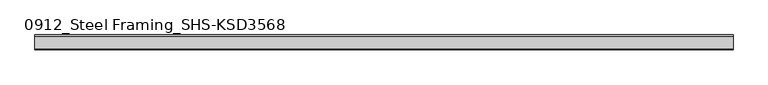
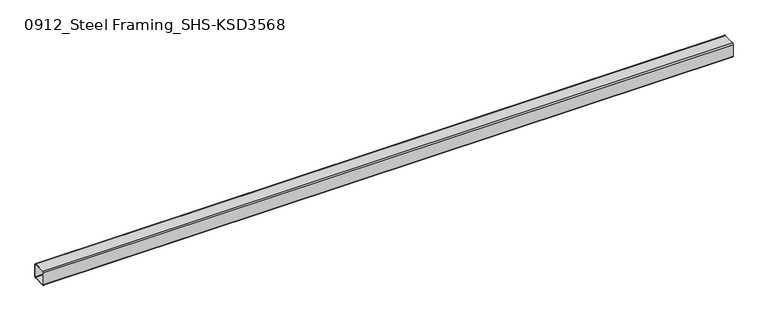
"""IFC4 building model written with IfcOpenShell, lengths in millimetres: beam geometry, 0912_Steel Framing_SHS-KSD3568 : H_SB_ASB_SHS-150x150x6."""

from ifc_helpers import new_model, si_unit, point, frame, frame_2d, origin, place, context, project, spatial, polyline, circle_curve, trimmed, segment, composite_curve, outline, extrude, source, transform, mapped, element, save


def beam_0912_steel_framing_shs_ksd3568_74c151f8(model_context):
    return source(origin(), model_context, "Body", "SweptSolid", [
        extrude(outline(composite_curve([segment(polyline([(75.0, 63.0), (75.0, -63.0)]), True, "CONTINUOUS"), segment(trimmed(circle_curve(frame_2d((63.0, -63.0)), 12.0), [point((75.0, -63.0))], [point((63.0, -75.0))], False, "CARTESIAN"), True, "CONTINUOUS"), segment(polyline([(63.0, -75.0), (-63.0, -75.0)]), True, "CONTINUOUS"), segment(trimmed(circle_curve(frame_2d((-63.0, -63.0)), 12.0), [point((-63.0, -75.0))], [point((-75.0, -63.0))], False, "CARTESIAN"), True, "CONTINUOUS"), segment(polyline([(-75.0, -63.0), (-75.0, 63.0)]), True, "CONTINUOUS"), segment(trimmed(circle_curve(frame_2d((-63.0, 63.0)), 12.0), [point((-75.0, 63.0))], [point((-63.0, 75.0))], False, "CARTESIAN"), True, "CONTINUOUS"), segment(polyline([(-63.0, 75.0), (63.0, 75.0)]), True, "CONTINUOUS"), segment(trimmed(circle_curve(frame_2d((63.0, 63.0)), 12.0), [point((63.0, 75.0))], [point((75.0, 63.0))], False, "CARTESIAN"), True, "CONTINUOUS")], self_intersect=False), holes=[composite_curve([segment(trimmed(circle_curve(frame_2d((-63.0, 63.0)), 6.0), [point((-63.0, 69.0))], [point((-69.0, 63.0))], True, "CARTESIAN"), True, "CONTINUOUS"), segment(polyline([(-69.0, 63.0), (-69.0, -63.0)]), True, "CONTINUOUS"), segment(trimmed(circle_curve(frame_2d((-63.0, -63.0)), 6.0), [point((-69.0, -63.0))], [point((-63.0, -69.0))], True, "CARTESIAN"), True, "CONTINUOUS"), segment(polyline([(-63.0, -69.0), (63.0, -69.0)]), True, "CONTINUOUS"), segment(trimmed(circle_curve(frame_2d((63.0, -63.0)), 6.0), [point((63.0, -69.0))], [point((69.0, -63.0))], True, "CARTESIAN"), True, "CONTINUOUS"), segment(polyline([(69.0, -63.0), (69.0, 63.0)]), True, "CONTINUOUS"), segment(trimmed(circle_curve(frame_2d((63.0, 63.0)), 6.0), [point((69.0, 63.0))], [point((63.0, 69.0))], True, "CARTESIAN"), True, "CONTINUOUS"), segment(polyline([(63.0, 69.0), (-63.0, 69.0)]), True, "CONTINUOUS")], self_intersect=False)]), frame((-3490.0, 0.0, 0.0), z_axis=(1.0, 0.0, 0.0), x_axis=(0.0, 1.0, 0.0)), (0.0, 0.0, 1.0), 6980.0),
    ])


if __name__ == "__main__":
    model = new_model("IFC4")
    model_context = context("Model", 3, world=origin())
    ifc_project = project(units=[si_unit("LENGTHUNIT", "METRE", prefix="MILLI")], contexts=[model_context])
    site = spatial("IfcSite", under=ifc_project)
    building = spatial("IfcBuilding", under=site)
    placement = place(None, origin())
    beam_0912_steel_framing_shs_ksd3568_shape = beam_0912_steel_framing_shs_ksd3568_74c151f8(model_context)
    element("IfcBeam", 1, ObjectType="0912_Steel Framing_SHS-KSD3568 : H_SB_ASB_SHS-150x150x6", at=placement, inside=building, context=model_context, shape_type="MappedRepresentation", body=[
        mapped(beam_0912_steel_framing_shs_ksd3568_shape, transform((0.0, 0.0, 0.0), x_axis=(1.0, 0.0, 0.0), y_axis=(0.0, 1.0, 0.0), z_axis=(0.0, 0.0, 1.0))),
    ])
    save(model, "model.ifc")

# Revit data of these elements
# Type "0912_Steel Framing_SHS-KSD3568 : H_SB_ASB_SHS-150x150x6"
#   H_WM Code_1 = "S01AA002-00001 | Main Steel Structure Fabrication Work | Shelter/Building | Medium Steel - Standard (90KG/M>Weight≥30KG/M) | Material: (   )"
#   H_WM Code_2 = "S03AA028-00001 | Main Steel Structure Erection Work | Shelter/Building | Medium Steel (90KG/M>Weight≥30KG/M) | Material: (   )"
#   H_WM Code_3 = "S01AA010-00001 | Main Steel Structure Fabrication Work | Shelter/Building | Steel Painting/Coating | for Non-Fireproofed Steel Surface, Surface Preparation, Primer, Second & Final Coat | Material: (   )"
#   H_Q'ty Cal Type Tag = "SB-Q2"
#   Perimeter = 0.60 m²/m
#   Nominal Weight = 26.40 kgf/m
#   Length [instance default] = 1.0000 m
#   b = 0.1500 m
#   h = 0.1500 m
#   tr = 0.0120 m
#   t = 0.0060 m
#   A = 28.36 m²
#   Structural Material [instance default] = Steel, 45-345
# Element 1 (IfcBeam, "0912_Steel Framing_SHS-KSD3568 : H_SB_ASB_SHS-150x150x6")
#   Structural Material = none
# Materials
#   "Steel, 45-345": class "Metal", colour RGB 189 187 185, transparency 0, Description = "Steel 345 MPa", Cost = 0
